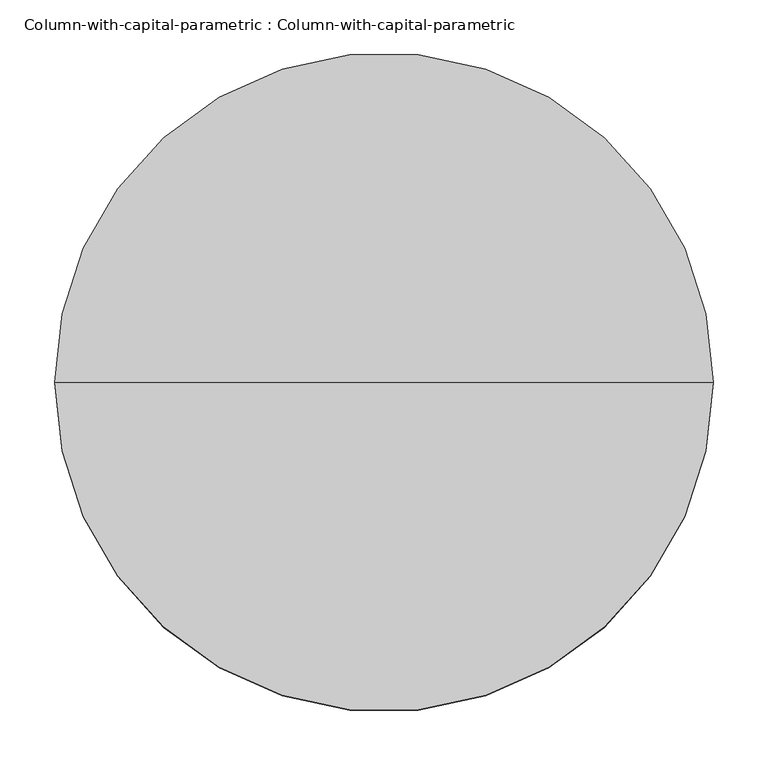
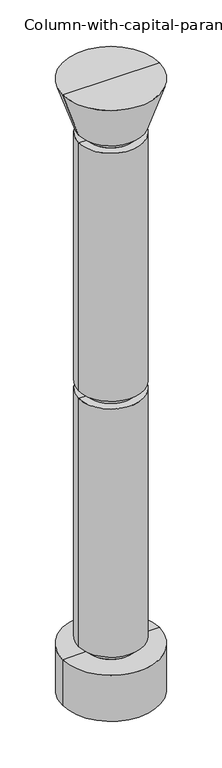
"""IFC4 building model written with IfcOpenShell, lengths in millimetres: column geometry, Column-with-capital-parametric : Column-with-capital-parametric."""

from ifc_helpers import new_model, si_unit, frame, origin, origin_with_axes, place, context, project, spatial, polyline, circle_curve, source, transform, mapped, element, save
from ifc_brep_helpers import plane_surface, cylinder_surface, revolved_surface, advanced_brep


def column_with_capital_parametric_column_with_capital_56f4d1e8(model_context):
    return source(origin(), model_context, "Body", "AdvancedBrep", [
        advanced_brep(
        [(-300.0, 0.0, 300.0), (300.0, 0.0, 300.0), (300.0, 0.0, 0.0), (-300.0, 0.0, 0.0), (0.0, 0.0, 0.0), (-150.0, 0.0, 300.0), (150.0, 0.0, 300.0), (-150.0, 0.0, 350.0), (150.0, 0.0, 350.0), (-200.0, 0.0, 350.0), (200.0, 0.0, 350.0), (-200.0, 0.0, 1975.0), (200.0, 0.0, 1975.0), (0.0, 0.0, 4000.0), (300.0, 0.0, 4000.0), (-300.0, 0.0, 4000.0), (200.0, 0.0, 3700.0), (-200.0, 0.0, 3700.0), (-150.0, 0.0, 3650.0), (150.0, 0.0, 3650.0), (200.0, 0.0, 3650.0), (-200.0, 0.0, 3650.0), (200.0, 0.0, 2025.0), (-200.0, 0.0, 2025.0), (-150.0, 0.0, 3700.0), (150.0, 0.0, 3700.0), (-150.0, 0.0, 1975.0), (150.0, 0.0, 1975.0), (-150.0, 0.0, 2025.0), (150.0, 0.0, 2025.0)],
        [
            (0, 1, circle_curve(frame((0.0, 0.0, 300.0), z_axis=(0.0, 0.0, -1.0), x_axis=(1.0, 0.0, 0.0)), 300.0)),
            (1, 2),
            (2, 3, circle_curve(origin_with_axes(), 300.0)),
            (3, 0),
            (2, 4),
            (4, 3),
            (2, 3, circle_curve(frame((0.0, 0.0, 0.0), z_axis=(0.0, 0.0, -1.0), x_axis=(1.0, 0.0, 0.0)), 300.0)),
            (1, 0, circle_curve(frame((0.0, 0.0, 300.0), z_axis=(0.0, 0.0, -1.0), x_axis=(1.0, 0.0, 0.0)), 300.0)),
            (5, 6, circle_curve(frame((0.0, 0.0, 300.0), z_axis=(0.0, 0.0, -1.0), x_axis=(1.0, 0.0, 0.0)), 150.0)),
            (6, 1),
            (0, 5),
            (6, 5, circle_curve(frame((0.0, 0.0, 300.0), z_axis=(0.0, 0.0, -1.0), x_axis=(1.0, 0.0, 0.0)), 150.0)),
            (7, 8, circle_curve(frame((0.0, 0.0, 350.0), z_axis=(0.0, 0.0, -1.0), x_axis=(1.0, 0.0, 0.0)), 150.0)),
            (8, 6),
            (5, 7),
            (8, 7, circle_curve(frame((0.0, 0.0, 350.0), z_axis=(0.0, 0.0, -1.0), x_axis=(1.0, 0.0, 0.0)), 150.0)),
            (9, 10, circle_curve(frame((0.0, 0.0, 350.0), z_axis=(0.0, 0.0, -1.0), x_axis=(1.0, 0.0, 0.0)), 200.0)),
            (10, 8),
            (7, 9),
            (10, 9, circle_curve(frame((0.0, 0.0, 350.0), z_axis=(0.0, 0.0, -1.0), x_axis=(1.0, 0.0, 0.0)), 200.0)),
            (11, 12, circle_curve(frame((0.0, 0.0, 1975.0), z_axis=(0.0, 0.0, -1.0), x_axis=(1.0, 0.0, 0.0)), 200.0)),
            (12, 10),
            (9, 11),
            (12, 11, circle_curve(frame((0.0, 0.0, 1975.0), z_axis=(0.0, 0.0, -1.0), x_axis=(1.0, 0.0, 0.0)), 200.0)),
            (13, 14),
            (14, 15, circle_curve(frame((0.0, 0.0, 4000.0), z_axis=(0.0, 0.0, 1.0), x_axis=(1.0, 0.0, 0.0)), 300.0)),
            (15, 13),
            (15, 14, circle_curve(frame((0.0, 0.0, 4000.0), z_axis=(0.0, 0.0, 1.0), x_axis=(1.0, 0.0, 0.0)), 300.0)),
            (14, 16),
            (16, 17, circle_curve(frame((0.0, 0.0, 3700.0), z_axis=(0.0, 0.0, 1.0), x_axis=(1.0, 0.0, 0.0)), 200.0)),
            (17, 15),
            (17, 16, circle_curve(frame((0.0, 0.0, 3700.0), z_axis=(0.0, 0.0, 1.0), x_axis=(1.0, 0.0, 0.0)), 200.0)),
            (18, 19, circle_curve(frame((0.0, 0.0, 3650.0), z_axis=(0.0, 0.0, -1.0), x_axis=(1.0, 0.0, 0.0)), 150.0)),
            (19, 20),
            (20, 21, circle_curve(frame((0.0, 0.0, 3650.0), z_axis=(0.0, 0.0, 1.0), x_axis=(1.0, 0.0, 0.0)), 200.0)),
            (21, 18),
            (20, 22),
            (22, 23, circle_curve(frame((0.0, 0.0, 2025.0), z_axis=(0.0, 0.0, 1.0), x_axis=(1.0, 0.0, 0.0)), 200.0)),
            (23, 21),
            (20, 21, circle_curve(frame((0.0, 0.0, 3650.0), z_axis=(0.0, 0.0, -1.0), x_axis=(1.0, 0.0, 0.0)), 200.0)),
            (23, 22, circle_curve(frame((0.0, 0.0, 2025.0), z_axis=(0.0, 0.0, 1.0), x_axis=(1.0, 0.0, 0.0)), 200.0)),
            (19, 18, circle_curve(frame((0.0, 0.0, 3650.0), z_axis=(0.0, 0.0, -1.0), x_axis=(1.0, 0.0, 0.0)), 150.0)),
            (24, 25, circle_curve(frame((0.0, 0.0, 3700.0), z_axis=(0.0, 0.0, -1.0), x_axis=(1.0, 0.0, 0.0)), 150.0)),
            (25, 19),
            (18, 24),
            (25, 24, circle_curve(frame((0.0, 0.0, 3700.0), z_axis=(0.0, 0.0, -1.0), x_axis=(1.0, 0.0, 0.0)), 150.0)),
            (16, 25),
            (24, 17),
            (26, 27, circle_curve(frame((0.0, 0.0, 1975.0), z_axis=(0.0, 0.0, -1.0), x_axis=(1.0, 0.0, 0.0)), 150.0)),
            (27, 12),
            (11, 26),
            (27, 26, circle_curve(frame((0.0, 0.0, 1975.0), z_axis=(0.0, 0.0, -1.0), x_axis=(1.0, 0.0, 0.0)), 150.0)),
            (28, 29, circle_curve(frame((0.0, 0.0, 2025.0), z_axis=(0.0, 0.0, -1.0), x_axis=(1.0, 0.0, 0.0)), 150.0)),
            (29, 27),
            (26, 28),
            (29, 28, circle_curve(frame((0.0, 0.0, 2025.0), z_axis=(0.0, 0.0, -1.0), x_axis=(1.0, 0.0, 0.0)), 150.0)),
            (22, 29),
            (28, 23),
        ],
        [
            cylinder_surface(frame((0.0, 0.0, 4203.0565088), z_axis=(0.0, 0.0, 1.0), x_axis=(1.0, 0.0, 0.0)), 300.0),
            plane_surface(frame((0.0, 0.0, 0.0), z_axis=(0.0, 0.0, -1.0), x_axis=(1.0, 0.0, 0.0))),
            plane_surface(frame((0.0, 0.0, 300.0), z_axis=(0.0, 0.0, 1.0), x_axis=(1.0, 0.0, 0.0))),
            cylinder_surface(frame((0.0, 0.0, 4203.0565088), z_axis=(0.0, 0.0, 1.0), x_axis=(1.0, 0.0, 0.0)), 150.0),
            plane_surface(frame((0.0, 0.0, 350.0), z_axis=(0.0, 0.0, -1.0), x_axis=(1.0, 0.0, 0.0))),
            cylinder_surface(frame((0.0, 0.0, 4203.0565088), z_axis=(0.0, 0.0, 1.0), x_axis=(1.0, 0.0, 0.0)), 200.0),
            plane_surface(frame((0.0, 0.0, 4000.0), z_axis=(0.0, 0.0, 1.0), x_axis=(1.0, 0.0, 0.0))),
            revolved_surface(polyline([(200.0, 0.0, 3700.0), (300.0, 0.0, 4000.0)]), (0.0, 0.0, 4203.0565088), (0.0, 0.0, 1.0)),
            plane_surface(frame((0.0, 0.0, 3650.0), z_axis=(0.0, 0.0, 1.0), x_axis=(1.0, 0.0, 0.0))),
            plane_surface(frame((0.0, 0.0, 3700.0), z_axis=(0.0, 0.0, -1.0), x_axis=(1.0, 0.0, 0.0))),
            plane_surface(frame((0.0, 0.0, 1975.0), z_axis=(0.0, 0.0, 1.0), x_axis=(1.0, 0.0, 0.0))),
            plane_surface(frame((0.0, 0.0, 2025.0), z_axis=(0.0, 0.0, -1.0), x_axis=(1.0, 0.0, 0.0))),
        ],
        [
            (0, [[1, 2, 3, 4]]),
            (1, [[-3, 5, 6]]),
            (1, [[7, -6, -5]]),
            (0, [[8, -4, -7, -2]]),
            (2, [[9, 10, -1, 11]]),
            (2, [[12, -11, -8, -10]]),
            (3, [[13, 14, -9, 15]]),
            (3, [[16, -15, -12, -14]]),
            (4, [[17, 18, -13, 19]]),
            (4, [[20, -19, -16, -18]]),
            (5, [[21, 22, -17, 23]]),
            (5, [[24, -23, -20, -22]]),
            (6, [[25, 26, 27]]),
            (6, [[-27, 28, -25]]),
            (7, [[-26, 29, 30, 31]]),
            (7, [[-28, -31, 32, -29]]),
            (8, [[33, 34, 35, 36]]),
            (5, [[-35, 37, 38, 39]]),
            (5, [[40, -39, 41, -37]]),
            (8, [[42, -36, -40, -34]]),
            (3, [[43, 44, -33, 45]]),
            (3, [[46, -45, -42, -44]]),
            (9, [[-30, 47, -43, 48]]),
            (9, [[-32, -48, -46, -47]]),
            (10, [[49, 50, -21, 51]]),
            (10, [[52, -51, -24, -50]]),
            (3, [[53, 54, -49, 55]]),
            (3, [[56, -55, -52, -54]]),
            (11, [[-38, 57, -53, 58]]),
            (11, [[-41, -58, -56, -57]]),
        ],
    ),
    ])


if __name__ == "__main__":
    model = new_model("IFC4")
    model_context = context("Model", 3, world=origin())
    ifc_project = project(units=[si_unit("LENGTHUNIT", "METRE", prefix="MILLI")], contexts=[model_context])
    site = spatial("IfcSite", under=ifc_project)
    building = spatial("IfcBuilding", under=site)
    placement = place(None, origin())
    column_with_capital_parametric_column_with_capital_shape = column_with_capital_parametric_column_with_capital_56f4d1e8(model_context)
    element("IfcColumn", 1, ObjectType="Column-with-capital-parametric : Column-with-capital-parametric", at=placement, inside=building, context=model_context, shape_type="MappedRepresentation", body=[
        mapped(column_with_capital_parametric_column_with_capital_shape, transform((0.0, 0.0, 0.0), x_axis=(1.0, 0.0, 0.0), y_axis=(0.0, 1.0, 0.0), z_axis=(0.0, 0.0, 1.0))),
    ])
    save(model, "model.ifc")

# Revit data of these elements
# Type "Column-with-capital-parametric : Column-with-capital-parametric"
#   Joint width = 50 mm
#   Diameter [instance default] = 600 mm
#   Capital height = 300 mm
#   Base height = 300 mm
